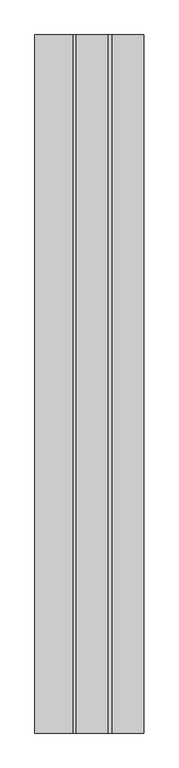
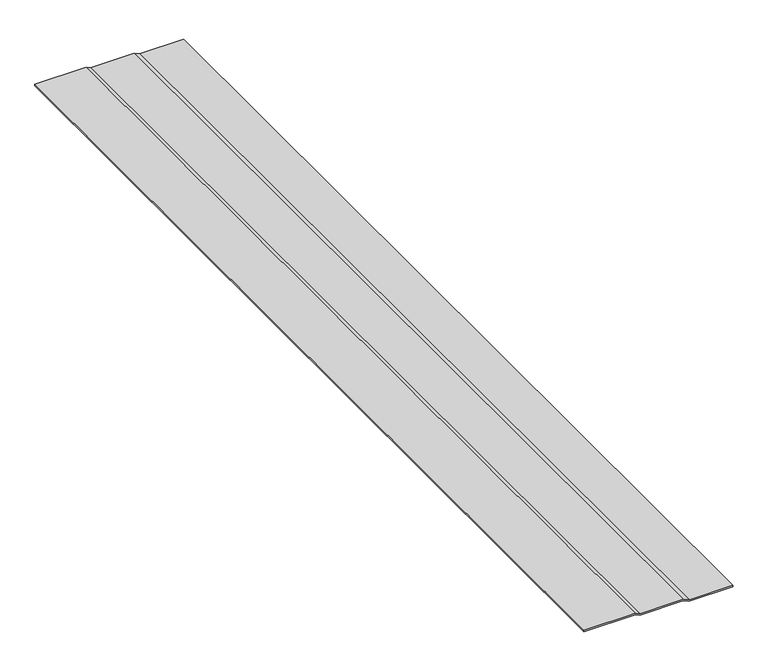
"""IFC4 building model written with IfcOpenShell, lengths in millimetres: proxy geometry, BITUMEN CAP SHEET 1:BITUMEN CAP SHEET 15300:299599 : BITUMEN CAP SHEET 1:BITUMEN CAP SHEET 15300:299599."""

from ifc_helpers import new_model, si_unit, frame, origin, place, context, project, spatial, polyline, outline, extrude, source, transform, mapped, element, save


def generic_models_9e2fcb59(model_context):
    return source(origin(), model_context, "Body", "SweptSolid", [
        extrude(outline(polyline([(40259.2002678, 2215.568251), (40259.2002678, 2307.7329126), (40262.3752679, 2307.7329126), (40262.3752679, 2216.213651), (40267.6612773, 2203.7488324), (40267.6612773, 2113.0650767), (40271.994072, 2103.3481752), (40271.994072, 1995.4616786), (40268.8188423, 1995.4616786), (40268.8188423, 2102.6728897), (40264.4862773, 2112.3892762), (40264.4862773, 2203.1034324), (40259.2002678, 2215.568251)])), frame((0.0, -774.5581163, 0.0), z_axis=(0.0, 1.0, 0.0), x_axis=(0.0, 0.0, 1.0)), (0.0, 0.0, 1.0), 2000.25),
    ])


if __name__ == "__main__":
    model = new_model("IFC4")
    model_context = context("Model", 3, world=origin())
    ifc_project = project(units=[si_unit("LENGTHUNIT", "METRE", prefix="MILLI")], contexts=[model_context])
    site = spatial("IfcSite", under=ifc_project)
    building = spatial("IfcBuilding", under=site)
    placement = place(None, origin())
    generic_models_shape = generic_models_9e2fcb59(model_context)
    element("IfcBuildingElementProxy", 1, Name="BITUMEN CAP SHEET 1:BITUMEN CAP SHEET 15300:299599 : BITUMEN CAP SHEET 1:BITUMEN CAP SHEET 15300:299599", ObjectType="BITUMEN CAP SHEET 1:BITUMEN CAP SHEET 15300:299599 : BITUMEN CAP SHEET 1:BITUMEN CAP SHEET 15300:299599", at=placement, inside=building, context=model_context, shape_type="MappedRepresentation", body=[
        mapped(generic_models_shape, transform((0.0, 0.0, 0.0), x_axis=(1.0, 0.0, 0.0), y_axis=(0.0, 1.0, 0.0), z_axis=(0.0, 0.0, 1.0))),
    ])
    save(model, "model.ifc")

# Revit data of these elements
# Type "BITUMEN CAP SHEET 1:BITUMEN CAP SHEET 15300:299599 : BITUMEN CAP SHEET 1:BITUMEN CAP SHEET 15300:299599"
#   NameOverride = "BITUMEN CAP SHEET 1:BITUMEN CAP SHEET 15300:299599"
#   ObjectTypeOverride = "BITUMEN CAP SHEET 1:BITUMEN CAP SHEET 15300"
#   Reference = "BITUMEN CAP SHEET 15300"
#   Category = "Generic Models"
#   Tag = "299599"
# Element 1 (IfcBuildingElementProxy, "BITUMEN CAP SHEET 1:BITUMEN CAP SHEET 15300:299599 : BITUMEN CAP SHEET 1:BITUMEN CAP SHEET 15300:299599")
#   Materials on its faces: "MODIFIED BITUMEN GRANULE SURFACED CAP SHEET"
# Materials
#   "MODIFIED BITUMEN GRANULE SURFACED CAP SHEET": class "Unassigned", colour RGB 85 85 127, transparency 0
